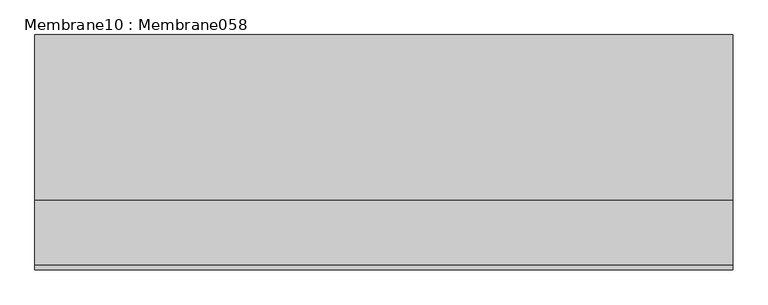
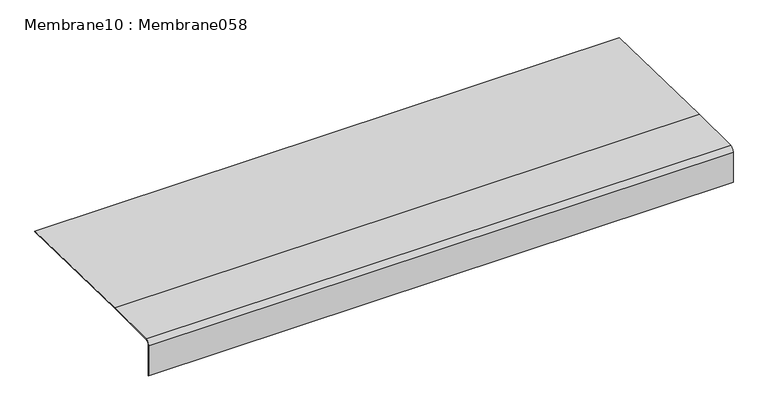
"""IFC4 building model written with IfcOpenShell, lengths in millimetres: proxy geometry, Membrane10 : Membrane058."""

import ifcopenshell
import ifcopenshell.guid

model = None  # the IFC model being written
_history = None  # IfcOwnerHistory: only IFC2X3 demands one
_inside = {}  # id of a spatial element -> (the spatial element, [elements in it])
_under = {}  # id of a project, library or spatial element -> (it, [spatial elements below it])
_declared = {}  # id of a project -> (the project, [libraries it declares])
_typed = {}  # id of a type object -> (the type object, [elements of that type])
_made_of = {}  # id of a material, layer set ... -> (it, [elements and type objects made of it])


def new_model(schema):
    """Start an empty IFC model of exactly this schema.

    Asked for "IFC4X3", IfcOpenShell would pick the latest addendum, in which some entities
    have other attributes; the version numbers below select the first issue.
    IFC2X3 requires an IfcOwnerHistory on every rooted entity: one is made here for all.
    """
    global model, _history
    if schema == "IFC4X3":
        model = ifcopenshell.file(schema_version=(4, 3, 0, 0))
    else:
        model = ifcopenshell.file(schema=schema)
    _inside.clear()
    _under.clear()
    _declared.clear()
    _typed.clear()
    _made_of.clear()
    _history = None
    if model.schema == "IFC2X3":
        org = make("IfcOrganization", Name="unknown")
        user = make(
            "IfcPersonAndOrganization",
            ThePerson=make("IfcPerson", FamilyName="unknown"),
            TheOrganization=org,
        )
        app = make(
            "IfcApplication",
            ApplicationDeveloper=org,
            Version="unknown",
            ApplicationFullName="unknown",
            ApplicationIdentifier="unknown",
        )
        _history = make(
            "IfcOwnerHistory",
            OwningUser=user,
            OwningApplication=app,
            ChangeAction="ADDED",
            CreationDate=0,
        )
    return model


def make(cls, **values):
    """One entity of the class cls with the attributes given. An attribute that is None is left unset."""
    return model.create_entity(
        cls, **{name: value for name, value in values.items() if value is not None}
    )


def rooted(cls, **values):
    """An entity with a GlobalId (a new one), such as an element, a storey or a relation."""
    return make(cls, GlobalId=ifcopenshell.guid.new(), OwnerHistory=_history, **values)


def si_unit(unit_type, name, prefix=None):
    """IfcSIUnit, for example si_unit("LENGTHUNIT", "METRE", prefix="MILLI")."""
    return make("IfcSIUnit", UnitType=unit_type, Prefix=prefix, Name=name)


def assignment(units):
    """IfcUnitAssignment: the units of a project."""
    return None if units is None else make("IfcUnitAssignment", Units=units)


def point(xyz):
    """IfcCartesianPoint."""
    return None if xyz is None else make("IfcCartesianPoint", Coordinates=xyz)


def direction(xyz):
    """IfcDirection."""
    return None if xyz is None else make("IfcDirection", DirectionRatios=xyz)


def frame(location, z_axis=None, x_axis=None):
    """IfcAxis2Placement3D, a coordinate frame: its origin and axes. An axis left out is left unset."""
    return make(
        "IfcAxis2Placement3D",
        Location=point(location),
        Axis=direction(z_axis),
        RefDirection=direction(x_axis),
    )


def frame_2d(location, x_axis=None):
    """IfcAxis2Placement2D, a coordinate frame in the plane: its origin and x axis."""
    return make(
        "IfcAxis2Placement2D", Location=point(location), RefDirection=direction(x_axis)
    )


def origin():
    """The frame at (0, 0, 0) with its axes left unset."""
    return frame((0.0, 0.0, 0.0))


def place(relative_to, where):
    """IfcLocalPlacement: puts the frame where relative to a parent placement (None: the world)."""
    return make(
        "IfcLocalPlacement", PlacementRelTo=relative_to, RelativePlacement=where
    )


def context(
    kind, dimensions, precision=None, world=None, true_north=None, identifier=None
):
    """IfcGeometricRepresentationContext, for example the 3D "Model" context."""
    return make(
        "IfcGeometricRepresentationContext",
        ContextIdentifier=identifier,
        ContextType=kind,
        CoordinateSpaceDimension=dimensions,
        Precision=precision,
        WorldCoordinateSystem=world,
        TrueNorth=true_north,
    )


def project(units=None, contexts=None):
    """IfcProject with its units and contexts."""
    return rooted(
        "IfcProject",
        Name="project",
        RepresentationContexts=contexts,
        UnitsInContext=assignment(units),
    )


def spatial(cls, under=None, at=None, **own):
    """A site, building, storey or space (cls), placed at a placement, below another one or the project."""
    s = rooted(cls, ObjectPlacement=at, **own)
    if under is not None:
        _under.setdefault(under.id(), (under, []))[1].append(s)
    return s


def polyline(points):
    """IfcPolyline through the points."""
    return make("IfcPolyline", Points=[point(p) for p in points])


def circle_curve(where, radius):
    """IfcCircle in the frame where."""
    return make("IfcCircle", Position=where, Radius=radius)


def trimmed(basis, trim1, trim2, sense, master):
    """IfcTrimmedCurve: the piece of a basis curve between two trims."""
    return make(
        "IfcTrimmedCurve",
        BasisCurve=basis,
        Trim1=trim1,
        Trim2=trim2,
        SenseAgreement=sense,
        MasterRepresentation=master,
    )


def segment(curve, same_sense, transition):
    """IfcCompositeCurveSegment."""
    return make(
        "IfcCompositeCurveSegment",
        Transition=transition,
        SameSense=same_sense,
        ParentCurve=curve,
    )


def composite_curve(segments, self_intersect=None):
    """IfcCompositeCurve: segments joined end to end."""
    return make("IfcCompositeCurve", Segments=segments, SelfIntersect=self_intersect)


def outline(outer, holes=None, kind="AREA"):
    """IfcArbitraryClosedProfileDef: a profile drawn as a closed curve; with holes, ...WithVoids."""
    if holes is None:
        return make("IfcArbitraryClosedProfileDef", ProfileType=kind, OuterCurve=outer)
    return make(
        "IfcArbitraryProfileDefWithVoids",
        ProfileType=kind,
        OuterCurve=outer,
        InnerCurves=holes,
    )


def extrude(swept, where, along, depth):
    """IfcExtrudedAreaSolid: the profile swept, set in the frame where, extruded along a direction by depth."""
    return make(
        "IfcExtrudedAreaSolid",
        SweptArea=swept,
        Position=where,
        ExtrudedDirection=direction(along),
        Depth=depth,
    )


def shape(context_of_items, identifier, shape_type, items):
    """IfcShapeRepresentation: the items that make up one representation, for example the "Body"."""
    return make(
        "IfcShapeRepresentation",
        ContextOfItems=context_of_items,
        RepresentationIdentifier=identifier,
        RepresentationType=shape_type,
        Items=items,
    )


def source(mapping_origin, context_of_items, identifier, shape_type, items):
    """IfcRepresentationMap: a shape defined once, which mapped items show again and again."""
    return make(
        "IfcRepresentationMap",
        MappingOrigin=mapping_origin,
        MappedRepresentation=shape(context_of_items, identifier, shape_type, items),
    )


def transform(
    local_origin,
    x_axis=None,
    y_axis=None,
    z_axis=None,
    scale=None,
    scale2=None,
    scale3=None,
    uniform=True,
):
    """IfcCartesianTransformationOperator3D, or its non-uniform kind. x_axis, y_axis, z_axis: its Axis1, 2, 3."""
    if uniform:
        return make(
            "IfcCartesianTransformationOperator3D",
            Axis1=direction(x_axis),
            Axis2=direction(y_axis),
            LocalOrigin=point(local_origin),
            Scale=scale,
            Axis3=direction(z_axis),
        )
    return make(
        "IfcCartesianTransformationOperator3DnonUniform",
        Axis1=direction(x_axis),
        Axis2=direction(y_axis),
        LocalOrigin=point(local_origin),
        Scale=scale,
        Axis3=direction(z_axis),
        Scale2=scale2,
        Scale3=scale3,
    )


def mapped(mapping_source, mapping_target):
    """IfcMappedItem: shows the shape of a source again, moved by a transform."""
    return make(
        "IfcMappedItem", MappingSource=mapping_source, MappingTarget=mapping_target
    )


def made_of(thing, what):
    """Note that an element or type object is made of a material, layer set ...; save() writes the relation."""
    if what is not None:
        _made_of.setdefault(what.id(), (what, []))[1].append(thing)
    return thing


def element(
    cls,
    number,
    at=None,
    inside=None,
    cuts=None,
    type_object=None,
    material=None,
    context=None,
    identifier="Body",
    shape_type=None,
    held_by="IfcProductDefinitionShape",
    body=None,
    shapes=None,
    **own,
):
    """One element of the class cls, such as IfcWall. Its Tag is "e" and its number.

    at: its placement. inside: the storey or other place that contains it. cuts: it is an
    opening in that element (IfcRelVoidsElement). A single representation is given by context,
    identifier, shape_type and body (its items); several are given by shapes. held_by: the class
    of the entity that holds the representations. save() writes the other relations.
    """
    e = rooted(cls, Tag="e%d" % number, ObjectPlacement=at, **own)
    if body is not None:
        shapes = [shape(context, identifier, shape_type, body)]
    if shapes is not None:
        e.Representation = make(held_by, Representations=shapes)
    if inside is not None:
        _inside.setdefault(inside.id(), (inside, []))[1].append(e)
    if cuts is not None:
        rooted(
            "IfcRelVoidsElement", RelatingBuildingElement=cuts, RelatedOpeningElement=e
        )
    if type_object is not None:
        _typed.setdefault(type_object.id(), (type_object, []))[1].append(e)
    return made_of(e, material)


def aggregate(whole, parts):
    """IfcRelAggregates: a whole, such as a stair, and the parts it consists of."""
    return rooted("IfcRelAggregates", RelatingObject=whole, RelatedObjects=parts)


def save(model, path):
    """Write the relations noted so far, then the file.

    IfcRelAggregates (storeys below a building ...), IfcRelContainedInSpatialStructure (elements
    in a storey), IfcRelDefinesByType, IfcRelAssociatesMaterial and IfcRelDeclares: one each for
    every whole, place, type object, material and project.
    """
    for whole, parts in _under.values():
        aggregate(whole, parts)
    for where, things in _inside.values():
        rooted(
            "IfcRelContainedInSpatialStructure",
            RelatedElements=things,
            RelatingStructure=where,
        )
    for kind, things in _typed.values():
        rooted("IfcRelDefinesByType", RelatedObjects=things, RelatingType=kind)
    for what, things in _made_of.values():
        rooted("IfcRelAssociatesMaterial", RelatedObjects=things, RelatingMaterial=what)
    for by, libraries in _declared.values():
        rooted("IfcRelDeclares", RelatingContext=by, RelatedDefinitions=libraries)
    model.write(path)


def membrane10_membrane058_abb4ba5d(model_context):
    return source(origin(), model_context, "Body", "SweptSolid", [
        extrude(outline(composite_curve([segment(polyline([(-5550.6165043, 40110.5621136), (-5552.6165043, 40110.5621136), (-5552.6165043, 40220.1581398)]), True, "CONTINUOUS"), segment(trimmed(circle_curve(frame_2d((-5537.6165043, 40220.1581398)), 15.0), [point((-5552.6165043, 40220.1581398))], [point((-5537.6165043, 40235.1581398))], False, "CARTESIAN"), True, "CONTINUOUS"), segment(polyline([(-5537.6165043, 40235.1581398), (-5351.7708809, 40235.1581398), (-4878.1775128, 40224.3228672), (-4878.2232585, 40222.3233905), (-5351.7937568, 40233.1581398), (-5537.6165043, 40233.1581398)]), True, "CONTINUOUS"), segment(trimmed(circle_curve(frame_2d((-5537.6165043, 40220.1581398)), 13.0), [point((-5537.6165043, 40233.1581398))], [point((-5550.6165043, 40220.1581398))], True, "CARTESIAN"), True, "CONTINUOUS"), segment(polyline([(-5550.6165043, 40220.1581398), (-5550.6165043, 40110.5621136)]), True, "CONTINUOUS")], self_intersect=False)), frame((12383.0178845, 0.0, 0.0), z_axis=(1.0, 0.0, 0.0), x_axis=(0.0, 1.0, 0.0)), (0.0, 0.0, 1.0), 2000.0),
    ])


if __name__ == "__main__":
    model = new_model("IFC4")
    model_context = context("Model", 3, world=origin())
    ifc_project = project(units=[si_unit("LENGTHUNIT", "METRE", prefix="MILLI")], contexts=[model_context])
    site = spatial("IfcSite", under=ifc_project)
    building = spatial("IfcBuilding", under=site)
    placement = place(None, origin())
    membrane10_membrane058_shape = membrane10_membrane058_abb4ba5d(model_context)
    element("IfcBuildingElementProxy", 1, Name="Membrane10 : Membrane058", ObjectType="Membrane10 : Membrane058", at=placement, inside=building, context=model_context, shape_type="MappedRepresentation", body=[
        mapped(membrane10_membrane058_shape, transform((0.0, 0.0, 0.0), x_axis=(1.0, 0.0, 0.0), y_axis=(0.0, 1.0, 0.0), z_axis=(0.0, 0.0, 1.0))),
    ])
    save(model, "model.ifc")

# Revit data of these elements
# Type "Membrane10 : Membrane058"
#   NameOverride = "Membrane058"
# Element 1 (IfcBuildingElementProxy, "Membrane10 : Membrane058")
#   Materials on its faces: "THREE PLY BUILT UP ROOF MEMBRANE"
# Materials
#   "THREE PLY BUILT UP ROOF MEMBRANE": class "Unassigned", colour RGB 63 63 63, transparency 0
